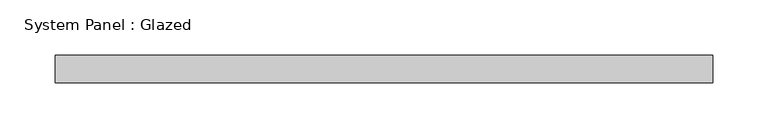
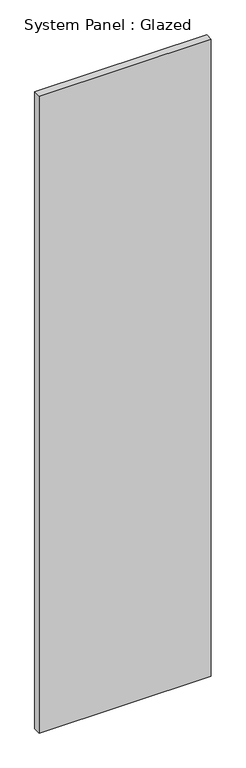
"""IFC4 building model written with IfcOpenShell, lengths in millimetres: plate geometry, System Panel : Glazed."""

from ifc_helpers import new_model, si_unit, origin, origin_with_axes, place, context, project, spatial, polyline, outline, extrude, source, transform, mapped, element, save


def system_panel_glazed_b202262a(model_context):
    return source(origin(), model_context, "Body", "SweptSolid", [
        extrude(outline(polyline([(297.5, 24.5), (-297.5, 24.5), (-297.5, 49.5), (297.5, 49.5), (297.5, 24.5)])), origin_with_axes(), (0.0, 0.0, 1.0), 2325.0),
    ])


if __name__ == "__main__":
    model = new_model("IFC4")
    model_context = context("Model", 3, world=origin())
    ifc_project = project(units=[si_unit("LENGTHUNIT", "METRE", prefix="MILLI")], contexts=[model_context])
    site = spatial("IfcSite", under=ifc_project)
    building = spatial("IfcBuilding", under=site)
    placement = place(None, origin())
    system_panel_glazed_shape = system_panel_glazed_b202262a(model_context)
    element("IfcPlate", 1, ObjectType="System Panel : Glazed", at=placement, inside=building, context=model_context, shape_type="MappedRepresentation", body=[
        mapped(system_panel_glazed_shape, transform((0.0, 0.0, 0.0), x_axis=(1.0, 0.0, 0.0), y_axis=(0.0, 1.0, 0.0), z_axis=(0.0, 0.0, 1.0))),
    ])
    save(model, "model.ifc")

# Revit data of these elements
# Element 1 (IfcPlate, "System Panel : Glazed")
#   Materials on its faces: "Glass"
# Materials
#   "Glass": class "Glass", colour RGB 0 128 192, transparency 0.9
